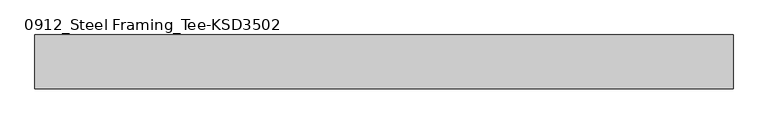
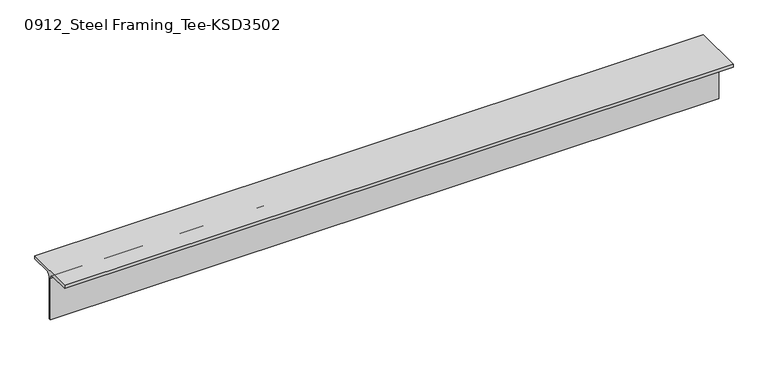
"""IFC4 building model written with IfcOpenShell, lengths in millimetres: member geometry, 0912_Steel Framing_Tee-KSD3502 : H_SB_ASB_CT-150x150x6.5x9."""

from ifc_helpers import new_model, si_unit, point, frame, frame_2d, origin, place, context, project, spatial, polyline, circle_curve, trimmed, segment, composite_curve, outline, extrude, source, transform, mapped, element, save


def member_0912_steel_framing_tee_ksd3502_928024c0(model_context):
    return source(origin(), model_context, "Body", "SweptSolid", [
        extrude(outline(composite_curve([segment(polyline([(-75.0, 75.0), (75.0, 75.0), (75.0, 66.0), (16.25, 66.0)]), True, "CONTINUOUS"), segment(trimmed(circle_curve(frame_2d((16.25, 53.0)), 13.0), [point((16.25, 66.0))], [point((3.25, 53.0))], True, "CARTESIAN"), True, "CONTINUOUS"), segment(polyline([(3.25, 53.0), (3.25, -75.0), (-3.25, -75.0), (-3.25, 53.0)]), True, "CONTINUOUS"), segment(trimmed(circle_curve(frame_2d((-16.25, 53.0)), 13.0), [point((-3.25, 53.0))], [point((-16.25, 66.0))], True, "CARTESIAN"), True, "CONTINUOUS"), segment(polyline([(-16.25, 66.0), (-75.0, 66.0), (-75.0, 75.0)]), True, "CONTINUOUS")], self_intersect=False)), frame((-983.95, 0.0, 0.0), z_axis=(1.0, 0.0, 0.0), x_axis=(0.0, 1.0, 0.0)), (0.0, 0.0, 1.0), 1951.2),
    ])


if __name__ == "__main__":
    model = new_model("IFC4")
    model_context = context("Model", 3, world=origin())
    ifc_project = project(units=[si_unit("LENGTHUNIT", "METRE", prefix="MILLI")], contexts=[model_context])
    site = spatial("IfcSite", under=ifc_project)
    building = spatial("IfcBuilding", under=site)
    placement = place(None, origin())
    member_0912_steel_framing_tee_ksd3502_shape = member_0912_steel_framing_tee_ksd3502_928024c0(model_context)
    element("IfcMember", 1, ObjectType="0912_Steel Framing_Tee-KSD3502 : H_SB_ASB_CT-150x150x6.5x9", at=placement, inside=building, context=model_context, shape_type="MappedRepresentation", body=[
        mapped(member_0912_steel_framing_tee_ksd3502_shape, transform((0.0, 0.0, 0.0), x_axis=(1.0, 0.0, 0.0), y_axis=(0.0, 1.0, 0.0), z_axis=(0.0, 0.0, 1.0))),
    ])
    save(model, "model.ifc")

# Revit data of these elements
# Type "0912_Steel Framing_Tee-KSD3502 : H_SB_ASB_CT-150x150x6.5x9"
#   H_WM Code_1 = "S01AA003-00001 | Main Steel Structure Fabrication Work | Shelter/Building | Light Steel - Standard (30KG/M>Weight) | Material: (   )"
#   H_WM Code_2 = "S03AA029-00001 | Main Steel Structure Erection Work | Shelter/Building | Light Steel (30KG/M>Weight) | Material: (   )"
#   H_WM Code_3 = "S01AA010-00001 | Main Steel Structure Fabrication Work | Shelter/Building | Steel Painting/Coating | for Non-Fireproofed Steel Surface, Surface Preparation, Primer, Second & Final Coat | Material: (   )"
#   H_Q'ty Cal Type Tag = "SB-Q2"
#   Width = 15.0 cm
#   Web Thickness = 0.65 cm
#   Web Fillet = 1.3 cm
#   Section Area = 23.39 cm²
#   Perimeter = 0.60 m²/m
#   Nominal Weight = 18.40 kgf/m
#   Height = 15.0 cm
#   Flange Thickness = 0.9 cm
#   Centroid Vertical = 7.5 cm
#   Centroid Horizontal = 7.5 cm
#   Length [instance default] = 1.5000 m
#   Structural Material [instance default] = Steel, 45-345
#   Warping Constant = (empty or 0)
#   Torsional Moment of Inertia = 0
#   Section Name Key = ""
#   Plastic Modulus weak axis = 0
#   Plastic Modulus strong axis = 0
#   Moment of Inertia weak axis = 0
#   Moment of Inertia strong axis = 0
#   Elastic Modulus weak axis = 0
#   Elastic Modulus strong axis = 0
#   Bolt Spacing = 0
#   Assembly Code = ""
# Element 1 (IfcMember, "0912_Steel Framing_Tee-KSD3502 : H_SB_ASB_CT-150x150x6.5x9")
#   Structural Material = none
# Materials
#   "Steel, 45-345": class "Metal", colour RGB 189 187 185, transparency 0, Description = "Steel 345 MPa", Cost = 0
